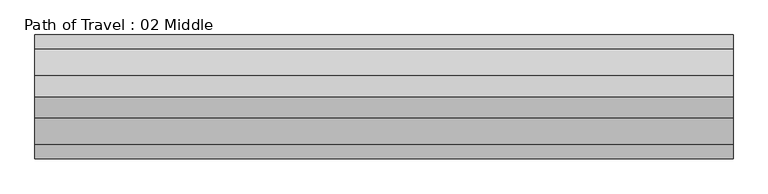
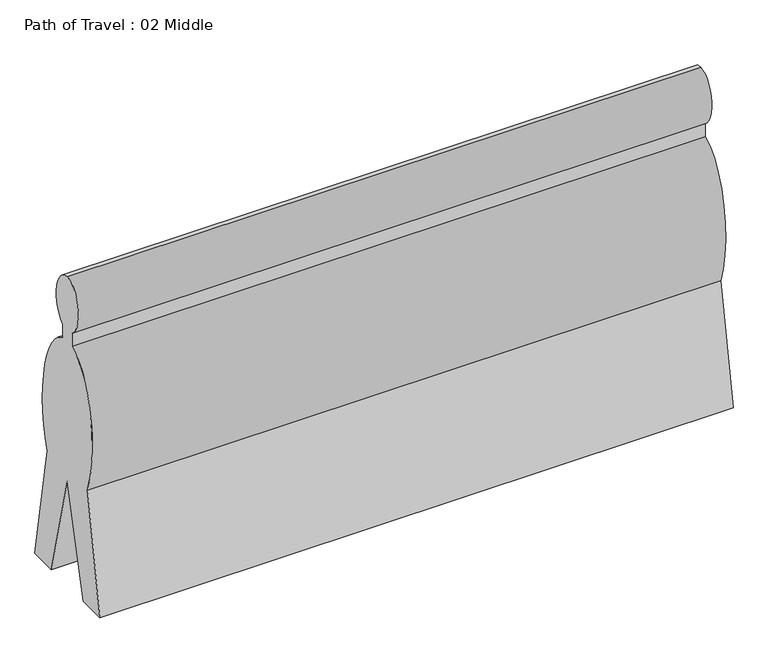
"""IFC4 building model written with IfcOpenShell, lengths in millimetres: proxy geometry, Path of Travel : 02 Middle."""

from ifc_helpers import new_model, si_unit, point, frame, origin, place, context, project, spatial, ellipse_curve, trimmed, source, transform, mapped, element, save
from ifc_brep_helpers import plane_surface, extruded_surface, advanced_brep


def path_of_travel_02_middle_3bd4d48d(model_context):
    return source(origin(), model_context, "Body", "AdvancedBrep", [
        advanced_brep(
        [(227.5554837, 0.0, 1727.2), (227.5554837, 42.9018657, 1436.6534209), (227.5554837, 42.9018657, 1363.4763406), (227.5554837, 184.1186263, 643.4144547), (227.5554837, 297.5699544, 0.0), (227.5554837, 145.6574193, 0.0), (227.5554837, 0.0, 584.2), (227.5554837, -145.6574193, 0.0), (227.5554837, -297.5699544, 0.0), (227.5554837, -184.1186263, 643.4144547), (227.5554837, -42.9018657, 1363.4763406), (227.5554837, -42.9018657, 1436.6534209), (3580.3554837, 0.0, 1727.2), (3580.3554837, -42.9018657, 1436.6534209), (3580.3554837, -42.9018657, 1363.4763406), (3580.3554837, -184.1186263, 643.4144547), (3580.3554837, -297.5699544, 0.0), (3580.3554837, -145.6574193, 0.0), (3580.3554837, 0.0, 584.2), (3580.3554837, 145.6574193, 0.0), (3580.3554837, 297.5699544, 0.0), (3580.3554837, 184.1186263, 643.4144547), (3580.3554837, 42.9018657, 1363.4763406), (3580.3554837, 42.9018657, 1436.6534209)],
        [
            (0, 1, ellipse_curve(frame((227.5554837, 0.0, 1574.8), z_axis=(-1.0, 0.0, 0.0), x_axis=(0.0, 0.0, 1.0)), 152.4, 101.6)),
            (1, 2),
            (2, 3, ellipse_curve(frame((227.5554837, 0.0, 914.4), z_axis=(-1.0, 0.0, 0.0), x_axis=(0.0, 0.0, -1.0)), 457.2, 228.6)),
            (3, 4),
            (4, 5),
            (5, 6),
            (6, 7),
            (7, 8),
            (8, 9),
            (9, 10, ellipse_curve(frame((227.5554837, 0.0, 914.4), z_axis=(-1.0, 0.0, 0.0), x_axis=(0.0, 0.0, -1.0)), 457.2, 228.6)),
            (10, 11),
            (11, 0, ellipse_curve(frame((227.5554837, 0.0, 1574.8), z_axis=(-1.0, 0.0, 0.0), x_axis=(0.0, 0.0, 1.0)), 152.4, 101.6)),
            (12, 13, ellipse_curve(frame((3580.3554837, 0.0, 1574.8), z_axis=(1.0, 0.0, 0.0), x_axis=(0.0, 0.0, 1.0)), 152.4, 101.6)),
            (13, 14),
            (14, 15, ellipse_curve(frame((3580.3554837, 0.0, 914.4), z_axis=(1.0, 0.0, 0.0), x_axis=(0.0, 0.0, -1.0)), 457.2, 228.6)),
            (15, 16),
            (16, 17),
            (17, 18),
            (18, 19),
            (19, 20),
            (20, 21),
            (21, 22, ellipse_curve(frame((3580.3554837, 0.0, 914.4), z_axis=(1.0, 0.0, 0.0), x_axis=(0.0, 0.0, -1.0)), 457.2, 228.6)),
            (22, 23),
            (23, 12, ellipse_curve(frame((3580.3554837, 0.0, 1574.8), z_axis=(1.0, 0.0, 0.0), x_axis=(0.0, 0.0, 1.0)), 152.4, 101.6)),
            (0, 12),
            (23, 1),
            (22, 2),
            (21, 3),
            (20, 4),
            (19, 5),
            (18, 6),
            (17, 7),
            (16, 8),
            (15, 9),
            (14, 10),
            (13, 11),
        ],
        [
            plane_surface(frame((227.5554837, 0.0, 0.0), z_axis=(-1.0, 0.0, 0.0), x_axis=(0.0, 0.0, 1.0))),
            plane_surface(frame((3580.3554837, 0.0, 0.0), z_axis=(1.0, 0.0, 0.0), x_axis=(0.0, 0.0, 1.0))),
            extruded_surface(trimmed(ellipse_curve(frame((3580.3554837, 0.0, 1574.8), z_axis=(-1.0, 0.0, 0.0), x_axis=(0.0, 0.0, 1.0)), 152.4, 101.6), [point((3580.3554837, 0.0, 1727.2))], [point((3580.3554837, 42.9018657, 1436.6534209))], True, "CARTESIAN"), (-3352.8, 0.0, 0.0), 3352.8),
            plane_surface(frame((227.5554837, 42.9018657, 1436.6534209), z_axis=(0.0, 1.0, 0.0), x_axis=(1.0, 0.0, 0.0))),
            extruded_surface(trimmed(ellipse_curve(frame((3580.3554837, 0.0, 914.4), z_axis=(-1.0, 0.0, 0.0), x_axis=(0.0, 0.0, -1.0)), 457.2, 228.6), [point((3580.3554837, 42.9018657, 1363.4763406))], [point((3580.3554837, 184.1186263, 643.4144547))], True, "CARTESIAN"), (-3352.8, 0.0, 0.0), 3352.8),
            plane_surface(frame((227.5554837, 184.1186263, 643.4144547), z_axis=(0.0, 0.9848077530122078, 0.17364817766693205), x_axis=(1.0, 0.0, 0.0))),
            plane_surface(frame((227.5554837, 297.5699544, 0.0), z_axis=(0.0, 0.0, -1.0), x_axis=(1.0, 0.0, 0.0))),
            plane_surface(frame((227.5554837, 145.6574193, 0.0), z_axis=(0.0, -0.9702957262760199, -0.2419218955995739), x_axis=(1.0, 0.0, 0.0))),
            plane_surface(frame((227.5554837, 0.0, 584.2), z_axis=(0.0, 0.9702957262759961, -0.24192189559966923), x_axis=(1.0, 0.0, 0.0))),
            plane_surface(frame((227.5554837, -145.6574193, 0.0), z_axis=(0.0, 0.0, -1.0), x_axis=(1.0, 0.0, 0.0))),
            plane_surface(frame((227.5554837, -297.5699544, 0.0), z_axis=(0.0, -0.984807753012208, 0.17364817766693066), x_axis=(1.0, 0.0, 0.0))),
            extruded_surface(trimmed(ellipse_curve(frame((3580.3554837, 0.0, 914.4), z_axis=(-1.0, 0.0, 0.0), x_axis=(0.0, 0.0, -1.0)), 457.2, 228.6), [point((3580.3554837, -184.1186263, 643.4144547))], [point((3580.3554837, -42.9018657, 1363.4763406))], True, "CARTESIAN"), (-3352.8, 0.0, 0.0), 3352.8),
            plane_surface(frame((227.5554837, -42.9018657, 1363.4763406), z_axis=(0.0, -1.0, 0.0), x_axis=(1.0, 0.0, 0.0))),
            extruded_surface(trimmed(ellipse_curve(frame((3580.3554837, 0.0, 1574.8), z_axis=(-1.0, 0.0, 0.0), x_axis=(0.0, 0.0, 1.0)), 152.4, 101.6), [point((3580.3554837, -42.9018657, 1436.6534209))], [point((3580.3554837, 0.0, 1727.2))], True, "CARTESIAN"), (-3352.8, 0.0, 0.0), 3352.8),
        ],
        [
            (0, [[1, 2, 3, 4, 5, 6, 7, 8, 9, 10, 11, 12]]),
            (1, [[13, 14, 15, 16, 17, 18, 19, 20, 21, 22, 23, 24]]),
            (2, [[-1, 25, -24, 26]]),
            (3, [[-2, -26, -23, 27]]),
            (4, [[-3, -27, -22, 28]]),
            (5, [[-4, -28, -21, 29]]),
            (6, [[-5, -29, -20, 30]]),
            (7, [[-6, -30, -19, 31]]),
            (8, [[-7, -31, -18, 32]]),
            (9, [[-8, -32, -17, 33]]),
            (10, [[-9, -33, -16, 34]]),
            (11, [[-10, -34, -15, 35]]),
            (12, [[-11, -35, -14, 36]]),
            (13, [[-12, -36, -13, -25]]),
        ],
    ),
    ])


if __name__ == "__main__":
    model = new_model("IFC4")
    model_context = context("Model", 3, world=origin())
    ifc_project = project(units=[si_unit("LENGTHUNIT", "METRE", prefix="MILLI")], contexts=[model_context])
    site = spatial("IfcSite", under=ifc_project)
    building = spatial("IfcBuilding", under=site)
    placement = place(None, origin())
    path_of_travel_02_middle_shape = path_of_travel_02_middle_3bd4d48d(model_context)
    element("IfcBuildingElementProxy", 1, Name="Path of Travel : 02 Middle", ObjectType="Path of Travel : 02 Middle", at=placement, inside=building, context=model_context, shape_type="MappedRepresentation", body=[
        mapped(path_of_travel_02_middle_shape, transform((0.0, 0.0, 0.0), x_axis=(1.0, 0.0, 0.0), y_axis=(0.0, 1.0, 0.0), z_axis=(0.0, 0.0, 1.0))),
    ])
    save(model, "model.ifc")

# Revit data of these elements
# Type "Path of Travel : 02 Middle"
#   Path of Egress [instance default] = 4' - 0"
#   built-in parameter 1001306 [instance default] = 4 (stored number, unit not read)
#   Dot at Start = no
#   Arrow in Middle = yes
#   Arrow at End = no
#   Egress Path = none
# Element 1 (IfcBuildingElementProxy, "Path of Travel : 02 Middle")
#   Path of Egress = 11' - 0"
#   built-in parameter 1001306 = 11 (stored number, unit not read)
#   Materials on its faces: "Egress Path Solid"
# Materials
#   "Egress Path Solid": class "Unassigned", colour RGB 255 128 64, transparency 0.75, Comments = "Rendering appearance not upgraded "
